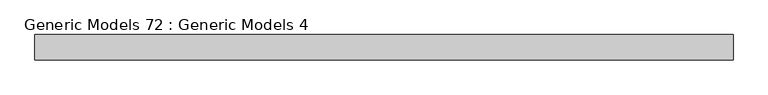
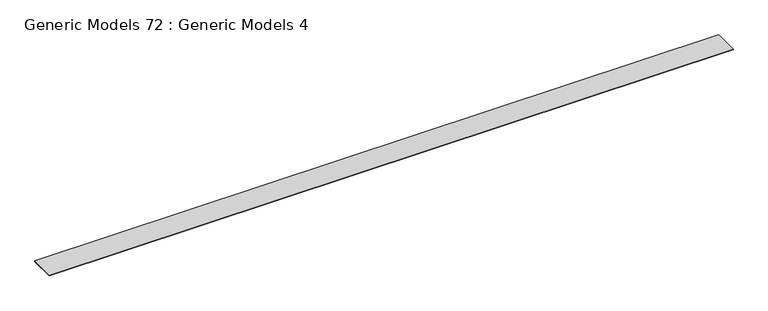
"""IFC4 building model written with IfcOpenShell, lengths in millimetres: proxy geometry, Generic Models 72 : Generic Models 4."""

from ifc_helpers import new_model, si_unit, frame, origin, place, context, project, spatial, polyline, outline, extrude, source, transform, mapped, element, save


def generic_models_72_generic_models_4_7d4b5bf1(model_context):
    return source(origin(), model_context, "Body", "SweptSolid", [
        extrude(outline(polyline([(21700.7658099, 13854.9341801), (21700.7658099, 13181.3246647), (3057.1658099, 13181.3246647), (3057.1658099, 13854.9341801), (21700.7658099, 13854.9341801)])), frame((0.0, 0.0, 129274.3086391), z_axis=(0.0, 0.0, 1.0), x_axis=(1.0, 0.0, 0.0)), (0.0, 0.0, 1.0), 18.3199747),
    ])


if __name__ == "__main__":
    model = new_model("IFC4")
    model_context = context("Model", 3, world=origin())
    ifc_project = project(units=[si_unit("LENGTHUNIT", "METRE", prefix="MILLI")], contexts=[model_context])
    site = spatial("IfcSite", under=ifc_project)
    building = spatial("IfcBuilding", under=site)
    placement = place(None, origin())
    generic_models_72_generic_models_4_shape = generic_models_72_generic_models_4_7d4b5bf1(model_context)
    element("IfcBuildingElementProxy", 1, Name="Generic Models 72 : Generic Models 4", ObjectType="Generic Models 72 : Generic Models 4", at=placement, inside=building, context=model_context, shape_type="MappedRepresentation", body=[
        mapped(generic_models_72_generic_models_4_shape, transform((0.0, 0.0, 0.0), x_axis=(1.0, 0.0, 0.0), y_axis=(0.0, 1.0, 0.0), z_axis=(0.0, 0.0, 1.0))),
    ])
    save(model, "model.ifc")

# Revit data of these elements
# Element 1 (IfcBuildingElementProxy, "Generic Models 72 : Generic Models 4")
#   Materials on its faces: "_5/8\" DRYWALL"
# Materials
#   "_5/8\" DRYWALL": class "Generic", colour RGB 191 191 191, transparency 0, Cost = 0
